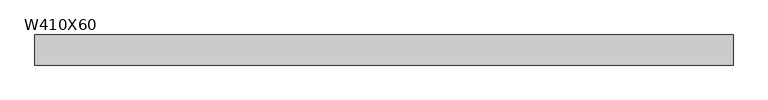
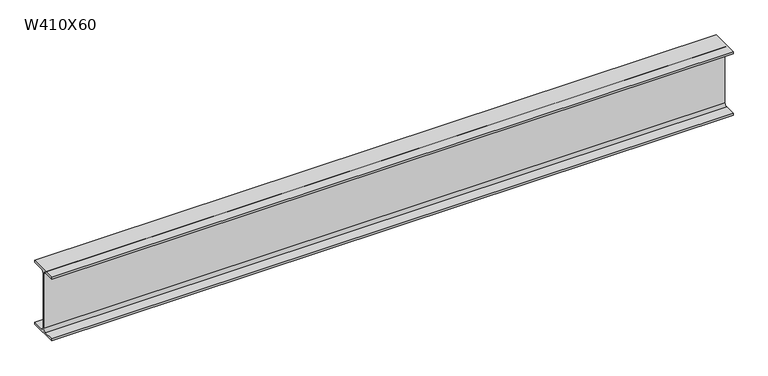
"""IFC4 building model written with IfcOpenShell, lengths in millimetres: beam geometry, M_W-Wide Flange : W410X60."""

import ifcopenshell
import ifcopenshell.guid

model = None  # the IFC model being written
_history = None  # IfcOwnerHistory: only IFC2X3 demands one
_inside = {}  # id of a spatial element -> (the spatial element, [elements in it])
_under = {}  # id of a project, library or spatial element -> (it, [spatial elements below it])
_declared = {}  # id of a project -> (the project, [libraries it declares])
_typed = {}  # id of a type object -> (the type object, [elements of that type])
_made_of = {}  # id of a material, layer set ... -> (it, [elements and type objects made of it])


def new_model(schema):
    """Start an empty IFC model of exactly this schema.

    Asked for "IFC4X3", IfcOpenShell would pick the latest addendum, in which some entities
    have other attributes; the version numbers below select the first issue.
    IFC2X3 requires an IfcOwnerHistory on every rooted entity: one is made here for all.
    """
    global model, _history
    if schema == "IFC4X3":
        model = ifcopenshell.file(schema_version=(4, 3, 0, 0))
    else:
        model = ifcopenshell.file(schema=schema)
    _inside.clear()
    _under.clear()
    _declared.clear()
    _typed.clear()
    _made_of.clear()
    _history = None
    if model.schema == "IFC2X3":
        org = make("IfcOrganization", Name="unknown")
        user = make(
            "IfcPersonAndOrganization",
            ThePerson=make("IfcPerson", FamilyName="unknown"),
            TheOrganization=org,
        )
        app = make(
            "IfcApplication",
            ApplicationDeveloper=org,
            Version="unknown",
            ApplicationFullName="unknown",
            ApplicationIdentifier="unknown",
        )
        _history = make(
            "IfcOwnerHistory",
            OwningUser=user,
            OwningApplication=app,
            ChangeAction="ADDED",
            CreationDate=0,
        )
    return model


def make(cls, **values):
    """One entity of the class cls with the attributes given. An attribute that is None is left unset."""
    return model.create_entity(
        cls, **{name: value for name, value in values.items() if value is not None}
    )


def rooted(cls, **values):
    """An entity with a GlobalId (a new one), such as an element, a storey or a relation."""
    return make(cls, GlobalId=ifcopenshell.guid.new(), OwnerHistory=_history, **values)


def si_unit(unit_type, name, prefix=None):
    """IfcSIUnit, for example si_unit("LENGTHUNIT", "METRE", prefix="MILLI")."""
    return make("IfcSIUnit", UnitType=unit_type, Prefix=prefix, Name=name)


def assignment(units):
    """IfcUnitAssignment: the units of a project."""
    return None if units is None else make("IfcUnitAssignment", Units=units)


def point(xyz):
    """IfcCartesianPoint."""
    return None if xyz is None else make("IfcCartesianPoint", Coordinates=xyz)


def direction(xyz):
    """IfcDirection."""
    return None if xyz is None else make("IfcDirection", DirectionRatios=xyz)


def frame(location, z_axis=None, x_axis=None):
    """IfcAxis2Placement3D, a coordinate frame: its origin and axes. An axis left out is left unset."""
    return make(
        "IfcAxis2Placement3D",
        Location=point(location),
        Axis=direction(z_axis),
        RefDirection=direction(x_axis),
    )


def frame_2d(location, x_axis=None):
    """IfcAxis2Placement2D, a coordinate frame in the plane: its origin and x axis."""
    return make(
        "IfcAxis2Placement2D", Location=point(location), RefDirection=direction(x_axis)
    )


def origin():
    """The frame at (0, 0, 0) with its axes left unset."""
    return frame((0.0, 0.0, 0.0))


def place(relative_to, where):
    """IfcLocalPlacement: puts the frame where relative to a parent placement (None: the world)."""
    return make(
        "IfcLocalPlacement", PlacementRelTo=relative_to, RelativePlacement=where
    )


def context(
    kind, dimensions, precision=None, world=None, true_north=None, identifier=None
):
    """IfcGeometricRepresentationContext, for example the 3D "Model" context."""
    return make(
        "IfcGeometricRepresentationContext",
        ContextIdentifier=identifier,
        ContextType=kind,
        CoordinateSpaceDimension=dimensions,
        Precision=precision,
        WorldCoordinateSystem=world,
        TrueNorth=true_north,
    )


def project(units=None, contexts=None):
    """IfcProject with its units and contexts."""
    return rooted(
        "IfcProject",
        Name="project",
        RepresentationContexts=contexts,
        UnitsInContext=assignment(units),
    )


def spatial(cls, under=None, at=None, **own):
    """A site, building, storey or space (cls), placed at a placement, below another one or the project."""
    s = rooted(cls, ObjectPlacement=at, **own)
    if under is not None:
        _under.setdefault(under.id(), (under, []))[1].append(s)
    return s


def polyline(points):
    """IfcPolyline through the points."""
    return make("IfcPolyline", Points=[point(p) for p in points])


def circle_curve(where, radius):
    """IfcCircle in the frame where."""
    return make("IfcCircle", Position=where, Radius=radius)


def trimmed(basis, trim1, trim2, sense, master):
    """IfcTrimmedCurve: the piece of a basis curve between two trims."""
    return make(
        "IfcTrimmedCurve",
        BasisCurve=basis,
        Trim1=trim1,
        Trim2=trim2,
        SenseAgreement=sense,
        MasterRepresentation=master,
    )


def segment(curve, same_sense, transition):
    """IfcCompositeCurveSegment."""
    return make(
        "IfcCompositeCurveSegment",
        Transition=transition,
        SameSense=same_sense,
        ParentCurve=curve,
    )


def composite_curve(segments, self_intersect=None):
    """IfcCompositeCurve: segments joined end to end."""
    return make("IfcCompositeCurve", Segments=segments, SelfIntersect=self_intersect)


def outline(outer, holes=None, kind="AREA"):
    """IfcArbitraryClosedProfileDef: a profile drawn as a closed curve; with holes, ...WithVoids."""
    if holes is None:
        return make("IfcArbitraryClosedProfileDef", ProfileType=kind, OuterCurve=outer)
    return make(
        "IfcArbitraryProfileDefWithVoids",
        ProfileType=kind,
        OuterCurve=outer,
        InnerCurves=holes,
    )


def extrude(swept, where, along, depth):
    """IfcExtrudedAreaSolid: the profile swept, set in the frame where, extruded along a direction by depth."""
    return make(
        "IfcExtrudedAreaSolid",
        SweptArea=swept,
        Position=where,
        ExtrudedDirection=direction(along),
        Depth=depth,
    )


def shape(context_of_items, identifier, shape_type, items):
    """IfcShapeRepresentation: the items that make up one representation, for example the "Body"."""
    return make(
        "IfcShapeRepresentation",
        ContextOfItems=context_of_items,
        RepresentationIdentifier=identifier,
        RepresentationType=shape_type,
        Items=items,
    )


def source(mapping_origin, context_of_items, identifier, shape_type, items):
    """IfcRepresentationMap: a shape defined once, which mapped items show again and again."""
    return make(
        "IfcRepresentationMap",
        MappingOrigin=mapping_origin,
        MappedRepresentation=shape(context_of_items, identifier, shape_type, items),
    )


def transform(
    local_origin,
    x_axis=None,
    y_axis=None,
    z_axis=None,
    scale=None,
    scale2=None,
    scale3=None,
    uniform=True,
):
    """IfcCartesianTransformationOperator3D, or its non-uniform kind. x_axis, y_axis, z_axis: its Axis1, 2, 3."""
    if uniform:
        return make(
            "IfcCartesianTransformationOperator3D",
            Axis1=direction(x_axis),
            Axis2=direction(y_axis),
            LocalOrigin=point(local_origin),
            Scale=scale,
            Axis3=direction(z_axis),
        )
    return make(
        "IfcCartesianTransformationOperator3DnonUniform",
        Axis1=direction(x_axis),
        Axis2=direction(y_axis),
        LocalOrigin=point(local_origin),
        Scale=scale,
        Axis3=direction(z_axis),
        Scale2=scale2,
        Scale3=scale3,
    )


def mapped(mapping_source, mapping_target):
    """IfcMappedItem: shows the shape of a source again, moved by a transform."""
    return make(
        "IfcMappedItem", MappingSource=mapping_source, MappingTarget=mapping_target
    )


def made_of(thing, what):
    """Note that an element or type object is made of a material, layer set ...; save() writes the relation."""
    if what is not None:
        _made_of.setdefault(what.id(), (what, []))[1].append(thing)
    return thing


def element(
    cls,
    number,
    at=None,
    inside=None,
    cuts=None,
    type_object=None,
    material=None,
    context=None,
    identifier="Body",
    shape_type=None,
    held_by="IfcProductDefinitionShape",
    body=None,
    shapes=None,
    **own,
):
    """One element of the class cls, such as IfcWall. Its Tag is "e" and its number.

    at: its placement. inside: the storey or other place that contains it. cuts: it is an
    opening in that element (IfcRelVoidsElement). A single representation is given by context,
    identifier, shape_type and body (its items); several are given by shapes. held_by: the class
    of the entity that holds the representations. save() writes the other relations.
    """
    e = rooted(cls, Tag="e%d" % number, ObjectPlacement=at, **own)
    if body is not None:
        shapes = [shape(context, identifier, shape_type, body)]
    if shapes is not None:
        e.Representation = make(held_by, Representations=shapes)
    if inside is not None:
        _inside.setdefault(inside.id(), (inside, []))[1].append(e)
    if cuts is not None:
        rooted(
            "IfcRelVoidsElement", RelatingBuildingElement=cuts, RelatedOpeningElement=e
        )
    if type_object is not None:
        _typed.setdefault(type_object.id(), (type_object, []))[1].append(e)
    return made_of(e, material)


def aggregate(whole, parts):
    """IfcRelAggregates: a whole, such as a stair, and the parts it consists of."""
    return rooted("IfcRelAggregates", RelatingObject=whole, RelatedObjects=parts)


def save(model, path):
    """Write the relations noted so far, then the file.

    IfcRelAggregates (storeys below a building ...), IfcRelContainedInSpatialStructure (elements
    in a storey), IfcRelDefinesByType, IfcRelAssociatesMaterial and IfcRelDeclares: one each for
    every whole, place, type object, material and project.
    """
    for whole, parts in _under.values():
        aggregate(whole, parts)
    for where, things in _inside.values():
        rooted(
            "IfcRelContainedInSpatialStructure",
            RelatedElements=things,
            RelatingStructure=where,
        )
    for kind, things in _typed.values():
        rooted("IfcRelDefinesByType", RelatedObjects=things, RelatingType=kind)
    for what, things in _made_of.values():
        rooted("IfcRelAssociatesMaterial", RelatedObjects=things, RelatingMaterial=what)
    for by, libraries in _declared.values():
        rooted("IfcRelDeclares", RelatingContext=by, RelatedDefinitions=libraries)
    model.write(path)


def w410x60_6fd633e1(model_context):
    return source(origin(), model_context, "Body", "SweptSolid", [
        extrude(outline(composite_curve([segment(polyline([(89.0, -190.7), (89.0, -203.5), (-89.0, -203.5), (-89.0, -190.7), (-21.05, -190.7)]), True, "CONTINUOUS"), segment(trimmed(circle_curve(frame_2d((-21.05, -173.5)), 17.2), [point((-21.05, -190.7))], [point((-3.85, -173.5))], True, "CARTESIAN"), True, "CONTINUOUS"), segment(polyline([(-3.85, -173.5), (-3.85, 173.5)]), True, "CONTINUOUS"), segment(trimmed(circle_curve(frame_2d((-21.05, 173.5)), 17.2), [point((-3.85, 173.5))], [point((-21.05, 190.7))], True, "CARTESIAN"), True, "CONTINUOUS"), segment(polyline([(-21.05, 190.7), (-89.0, 190.7), (-89.0, 203.5), (89.0, 203.5), (89.0, 190.7), (21.05, 190.7)]), True, "CONTINUOUS"), segment(trimmed(circle_curve(frame_2d((21.05, 173.5)), 17.2), [point((21.05, 190.7))], [point((3.85, 173.5))], True, "CARTESIAN"), True, "CONTINUOUS"), segment(polyline([(3.85, 173.5), (3.85, -173.5)]), True, "CONTINUOUS"), segment(trimmed(circle_curve(frame_2d((21.05, -173.5)), 17.2), [point((3.85, -173.5))], [point((21.05, -190.7))], True, "CARTESIAN"), True, "CONTINUOUS"), segment(polyline([(21.05, -190.7), (89.0, -190.7)]), True, "CONTINUOUS")], self_intersect=False)), frame((-2060.6399643, 0.0, 0.0), z_axis=(1.0, 0.0, 0.0), x_axis=(0.0, 1.0, 0.0)), (0.0, 0.0, 1.0), 4121.2799286),
    ])


if __name__ == "__main__":
    model = new_model("IFC4")
    model_context = context("Model", 3, world=origin())
    ifc_project = project(units=[si_unit("LENGTHUNIT", "METRE", prefix="MILLI")], contexts=[model_context])
    site = spatial("IfcSite", under=ifc_project)
    building = spatial("IfcBuilding", under=site)
    placement = place(None, origin())
    w410x60_shape = w410x60_6fd633e1(model_context)
    element("IfcBeam", 1, ObjectType="M_W-Wide Flange : W410X60", at=placement, inside=building, context=model_context, shape_type="MappedRepresentation", body=[
        mapped(w410x60_shape, transform((0.0, 0.0, 0.0), x_axis=(1.0, 0.0, 0.0), y_axis=(0.0, 1.0, 0.0), z_axis=(0.0, 0.0, 1.0))),
    ])
    save(model, "model.ifc")

# Revit data of these elements
# Type "M_W-Wide Flange : W410X60"
#   Manufacturer = "Manufacturer"
#   AccessibilityPerformance = "AccessibilityPerformance"
#   CodePerformance = "CodePerformance"
#   Color = "Color"
#   Constituents = "Constituents"
#   Features = "Features"
#   Finish = "Finish"
#   Grade = "Grade"
#   Material = "Material"
#   ModelReference = "ModelReference"
#   NominalHeight = "NominalHeight"
#   NominalLength = "NominalLength"
#   NominalWidth = "NominalWidth"
#   ProductionYear = "ProductionYear"
#   Reference = "Reference"
#   Shape = "Shape"
#   Size = "Size"
#   SustainabilityPerformance = "SustainabilityPerformance"
#   WarrantyDescription = "WarrantyDescription"
#   WarrantyDurationLabor = "WarrantyDurationLabor"
#   WarrantyDurationParts = "WarrantyDurationParts"
#   WarrantyGuarantorLabor = "WarrantyGuarantorLabor"
#   WarrantyGuarantorParts = "WarrantyGuarantorParts"
#   ExpectedLife = "ExpectedLife"
#   ReplacementCost = "ReplacementCost"
#   AssetAccountingType = "FIXED"
#   ModelLabel = "ModelLabel"
#   W = 0.58
#   Start Extension Calculation [instance default] = 3.000 m
#   Start Extension [instance default] = -0.0127 m
#   End Extension Calculation [instance default] = 3.000 m
#   End Extension [instance default] = -0.0127 m
#   Length [instance default] = 1.524 m
#   bf = 0.178 m
#   d = 0.407 m
#   k = 0.030 m
#   kr = 0.0172 m
#   tf = 0.0128 m
#   tw = 0.0077 m
#   A = 0.0076 m²
#   Structural Material [instance default] = Metal - Steel - 345 MPa
#   Assembly Code = ""
# Element 1 (IfcBeam, "M_W-Wide Flange : W410X60")
#   Materials on its faces: "Metal - Steel - 345 MPa"
# Materials
#   "Metal - Steel - 345 MPa": class "Metal", colour RGB 247 247 247, transparency 0
